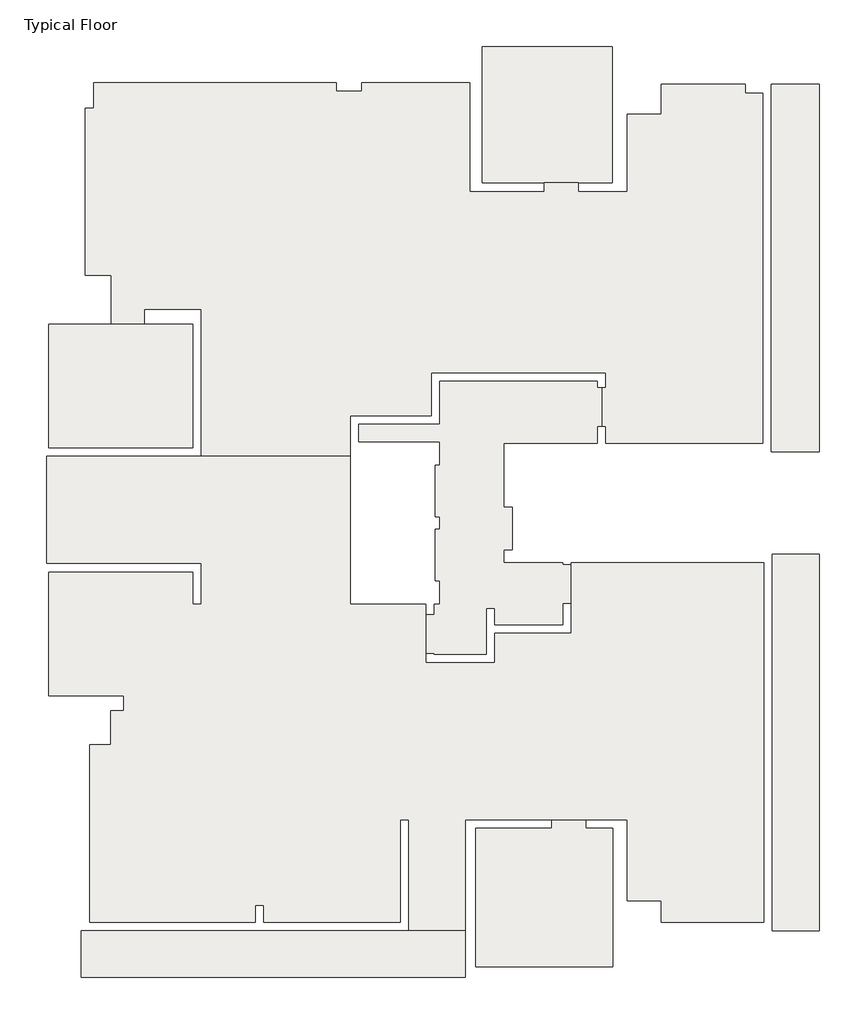
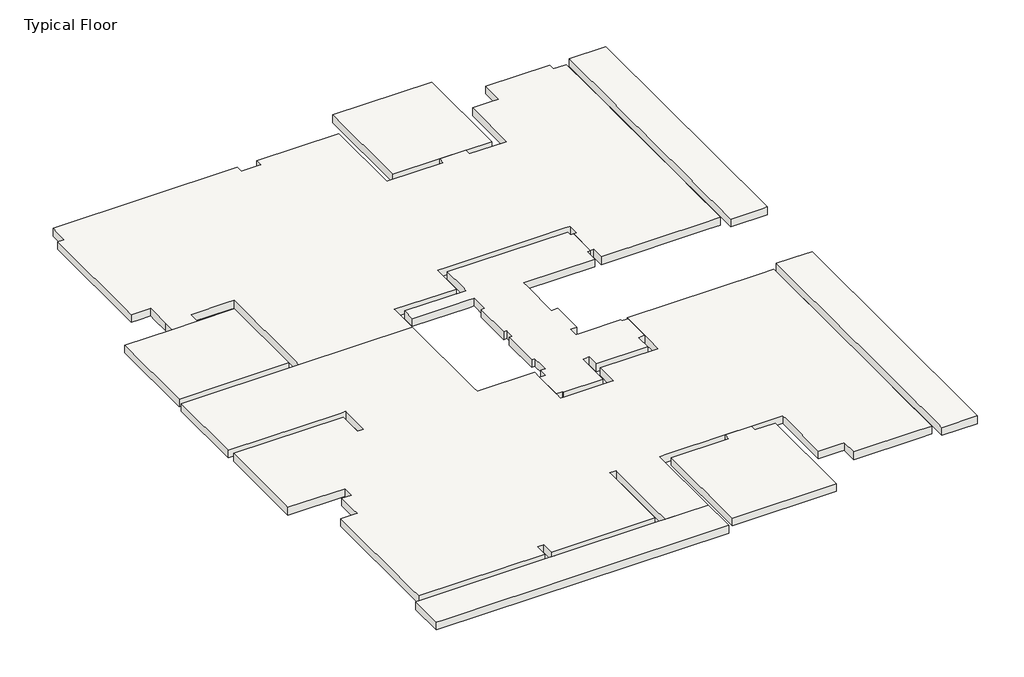
# One storey: 9 slabs.
"""IFC4 building model written with IfcOpenShell, lengths in millimetres."""

from ifc_helpers import new_model, si_unit, frame, origin, place, context, project, spatial, polyline, outline, extrude, faceted_brep, element, save

model = new_model("IFC4")

# Units and contexts
model_context = context("Model", 3, world=origin())
ifc_project = project(units=[si_unit("LENGTHUNIT", "METRE", prefix="MILLI")], contexts=[model_context])

# Site, building, storey
site = spatial("IfcSite", under=ifc_project)
building = spatial("IfcBuilding", under=site)
storey = spatial("IfcBuildingStorey", under=building, Name="Typical Floor", Elevation=3150.0)

# Slabs
placement = place(None, origin())
element("IfcSlab", 1, ObjectType="25", at=placement, inside=storey, context=model_context, shape_type="Brep", body=[
    faceted_brep([(1799.9138343, 9657.4646681, 2900.0), (1799.9138343, 6457.4646681, 2900.0), (1000.2209526, 6457.4646681, 2900.0), (199.8822614, 6457.4646681, 2900.0), (-1246.8886915, 6457.4646681, 2900.0), (-1246.8886915, 9657.4646681, 2900.0), (1799.9138343, 9657.4646681, 3150.0), (-1246.8886915, 9657.4646681, 3150.0), (-1246.8886915, 6457.4646681, 3150.0), (199.8822614, 6457.4646681, 3150.0), (1000.2209526, 6457.4646681, 3150.0), (1799.9138343, 6457.4646681, 3150.0)], [[[0, 1, 2, 3, 4, 5]], [[6, 7, 8, 9, 10, 11]], [[1, 0, 6, 11]], [[4, 3, 2, 1, 11, 10, 9, 8]], [[5, 4, 8, 7]], [[0, 5, 7, 6]]]),
])
element("IfcSlab", 2, ObjectType="25", at=placement, inside=storey, context=model_context, shape_type="Brep", body=[
    faceted_brep([(-8041.6160164, 3148.6252115, 2900.0), (-8041.6160164, 247.4292682, 2900.0), (-11417.5737279, 247.4292682, 2900.0), (-11417.5737279, 3148.6252115, 2900.0), (-9955.8228668, 3148.6252115, 2900.0), (-9181.8657294, 3148.6252115, 2900.0), (-8041.6160164, 3148.6252115, 3150.0), (-9181.8657294, 3148.6252115, 3150.0), (-9955.8228668, 3148.6252115, 3150.0), (-11417.5737279, 3148.6252115, 3150.0), (-11417.5737279, 247.4292682, 3150.0), (-8041.6160164, 247.4292682, 3150.0)], [[[0, 1, 2, 3, 4, 5]], [[6, 7, 8, 9, 10, 11]], [[1, 0, 6, 11]], [[2, 1, 11, 10]], [[3, 2, 10, 9]], [[0, 5, 4, 3, 9, 8, 7, 6]]]),
])
element("IfcSlab", 3, ObjectType="25", at=placement, inside=storey, context=model_context, shape_type="Brep", body=[
    faceted_brep([(-11467.5737279, -2465.8036059, 2900.0), (-11467.5737279, 47.4292682, 2900.0), (-7841.6160164, 47.4292682, 2900.0), (-4348.0741106, 47.4292682, 2900.0), (-4348.0741106, -3216.4704639, 2900.0), (-4348.0741106, -3416.4704639, 2900.0), (-2578.9868545, -3416.4704639, 2900.0), (-2578.9868545, -3670.5462389, 2900.0), (-2578.9868545, -4570.3979419, 2900.0), (-2578.9868545, -4796.9488413, 2900.0), (-2378.9868545, -4796.9488413, 2900.0), (-951.9279184, -4796.9488413, 2900.0), (-951.9279184, -4596.9488413, 2900.0), (-951.9279184, -4098.2404601, 2900.0), (833.928377, -4098.2404601, 2900.0), (833.928377, -3898.2404601, 2900.0), (833.928377, -3399.5320789, 2900.0), (833.928377, -2499.6803759, 2900.0), (833.928377, -2446.7479228, 2900.0), (4951.7310336, -2446.7479228, 2900.0), (5351.7310336, -2446.7479228, 2900.0), (5351.7310336, -10874.7377812, 2900.0), (4951.7310336, -10874.7377812, 2900.0), (2953.3437999, -10874.7377812, 2900.0), (2953.3437999, -10374.7377812, 2900.0), (2753.3437999, -10374.7377812, 2900.0), (2155.1912932, -10374.7377812, 2900.0), (2155.1912932, -8672.5783859, 2900.0), (2155.1912932, -8472.5783859, 2900.0), (1180.1912932, -8472.5783859, 2900.0), (379.852602, -8472.5783859, 2900.0), (-1396.4017034, -8472.5783859, 2900.0), (-1646.4017034, -8472.5783859, 2900.0), (-1646.4017034, -11075.5031849, 2900.0), (-2972.9736513, -11075.5031849, 2900.0), (-2972.9736513, -10475.5031849, 2900.0), (-2972.9736513, -9073.8910533, 2900.0), (-2972.9736513, -8473.8910533, 2900.0), (-3172.9736513, -8473.8910533, 2900.0), (-3172.9736513, -9073.8910533, 2900.0), (-3172.9736513, -10475.5031849, 2900.0), (-3172.9736513, -10874.7377812, 2900.0), (-6376.4457141, -10874.7377812, 2900.0), (-6376.4457141, -10475.5031849, 2900.0), (-6576.4457141, -10475.5031849, 2900.0), (-6576.4457141, -10874.7377812, 2900.0), (-10457.6225223, -10874.7377812, 2900.0), (-10457.6225223, -10475.5031849, 2900.0), (-10457.6225223, -6721.9995493, 2900.0), (-9957.6225223, -6721.9995493, 2900.0), (-9957.6225223, -6521.9995493, 2900.0), (-9957.6225223, -5916.9995493, 2900.0), (-9656.1405093, -5916.9995493, 2900.0), (-9656.1405093, -5566.9995493, 2900.0), (-11417.5737279, -5566.9995493, 2900.0), (-11417.5737279, -2665.8036059, 2900.0), (-8042.7593383, -2665.8036059, 2900.0), (-8042.7593383, -3416.4704639, 2900.0), (-7842.7593383, -3416.4704639, 2900.0), (-7842.7593383, -2465.8036059, 2900.0), (-8042.7593383, -2465.8036059, 2900.0), (-11467.5737279, 47.4292682, 3150.0), (-11467.5737279, -2465.8036059, 3150.0), (-8042.7593383, -2465.8036059, 3150.0), (-7842.7593383, -2465.8036059, 3150.0), (-7842.7593383, -3416.4704639, 3150.0), (-8042.7593383, -3416.4704639, 3150.0), (-8042.7593383, -2665.8036059, 3150.0), (-11417.5737279, -2665.8036059, 3150.0), (-11417.5737279, -5566.9995493, 3150.0), (-9656.1405093, -5566.9995493, 3150.0), (-9656.1405093, -5916.9995493, 3150.0), (-9957.6225223, -5916.9995493, 3150.0), (-9957.6225223, -6521.9995493, 3150.0), (-9957.6225223, -6721.9995493, 3150.0), (-10457.6225223, -6721.9995493, 3150.0), (-10457.6225223, -10475.5031849, 3150.0), (-10457.6225223, -10874.7377812, 3150.0), (-6576.4457141, -10874.7377812, 3150.0), (-6576.4457141, -10475.5031849, 3150.0), (-6376.4457141, -10475.5031849, 3150.0), (-6376.4457141, -10874.7377812, 3150.0), (-3172.9736513, -10874.7377812, 3150.0), (-3172.9736513, -10475.5031849, 3150.0), (-3172.9736513, -9073.8910533, 3150.0), (-3172.9736513, -8473.8910533, 3150.0), (-2972.9736513, -8473.8910533, 3150.0), (-2972.9736513, -9073.8910533, 3150.0), (-2972.9736513, -10475.5031849, 3150.0), (-2972.9736513, -11075.5031849, 3150.0), (-1646.4017034, -11075.5031849, 3150.0), (-1646.4017034, -8472.5783859, 3150.0), (-1396.4017034, -8472.5783859, 3150.0), (379.852602, -8472.5783859, 3150.0), (1180.1912932, -8472.5783859, 3150.0), (2155.1912932, -8472.5783859, 3150.0), (2155.1912932, -8672.5783859, 3150.0), (2155.1912932, -10374.7377812, 3150.0), (2753.3437999, -10374.7377812, 3150.0), (2953.3437999, -10374.7377812, 3150.0), (2953.3437999, -10874.7377812, 3150.0), (4951.7310336, -10874.7377812, 3150.0), (5351.7310336, -10874.7377812, 3150.0), (5351.7310336, -9023.8910533, 3150.0), (5351.7310336, -8523.8910533, 3150.0), (5351.7310336, -4555.4465944, 3150.0), (5351.7310336, -4055.4465944, 3150.0), (5351.7310336, -2446.7479228, 3150.0), (4951.7310336, -2446.7479228, 3150.0), (833.928377, -2446.7479228, 3150.0), (833.928377, -2499.6803759, 3150.0), (833.928377, -3399.5320789, 3150.0), (833.928377, -3898.2404601, 3150.0), (833.928377, -4098.2404601, 3150.0), (-951.9279184, -4098.2404601, 3150.0), (-951.9279184, -4596.9488413, 3150.0), (-951.9279184, -4796.9488413, 3150.0), (-2378.9868545, -4796.9488413, 3150.0), (-2578.9868545, -4796.9488413, 3150.0), (-2578.9868545, -4570.3979419, 3150.0), (-2578.9868545, -3670.5462389, 3150.0), (-2578.9868545, -3416.4704639, 3150.0), (-4348.0741106, -3416.4704639, 3150.0), (-4348.0741106, -3216.4704639, 3150.0), (-4348.0741106, 47.4292682, 3150.0), (-7841.6160164, 47.4292682, 3150.0)], [[[0, 1, 2, 3, 4, 5, 6, 7, 8, 9, 10, 11, 12, 13, 14, 15, 16, 17, 18, 19, 20, 21, 22, 23, 24, 25, 26, 27, 28, 29, 30, 31, 32, 33, 34, 35, 36, 37, 38, 39, 40, 41, 42, 43, 44, 45, 46, 47, 48, 49, 50, 51, 52, 53, 54, 55, 56, 57, 58, 59, 60]], [[61, 62, 63, 64, 65, 66, 67, 68, 69, 70, 71, 72, 73, 74, 75, 76, 77, 78, 79, 80, 81, 82, 83, 84, 85, 86, 87, 88, 89, 90, 91, 92, 93, 94, 95, 96, 97, 98, 99, 100, 101, 102, 103, 104, 105, 106, 107, 108, 109, 110, 111, 112, 113, 114, 115, 116, 117, 118, 119, 120, 121, 122, 123, 124, 125]], [[1, 0, 62, 61]], [[2, 1, 61, 125]], [[3, 2, 125, 124]], [[3, 124, 123, 122, 5, 4]], [[6, 5, 122, 121]], [[6, 121, 120, 119, 118, 9, 8, 7]], [[9, 118, 117, 116, 11, 10]], [[11, 116, 115, 114, 13, 12]], [[14, 13, 114, 113]], [[14, 113, 112, 111, 110, 109, 18, 17, 16, 15]], [[18, 109, 108, 107, 20, 19]], [[21, 20, 107, 106, 105, 104, 103, 102]], [[21, 102, 101, 100, 23, 22]], [[24, 23, 100, 99]], [[24, 99, 98, 97, 26, 25]], [[26, 97, 96, 95, 28, 27]], [[28, 95, 94, 93, 92, 91, 32, 31, 30, 29]], [[33, 32, 91, 90]], [[34, 33, 90, 89]], [[34, 89, 88, 87, 86, 37, 36, 35]], [[38, 37, 86, 85]], [[38, 85, 84, 83, 82, 41, 40, 39]], [[42, 41, 82, 81]], [[43, 42, 81, 80]], [[44, 43, 80, 79]], [[45, 44, 79, 78]], [[46, 45, 78, 77]], [[46, 77, 76, 75, 48, 47]], [[49, 48, 75, 74]], [[49, 74, 73, 72, 51, 50]], [[52, 51, 72, 71]], [[53, 52, 71, 70]], [[54, 53, 70, 69]], [[55, 54, 69, 68]], [[56, 55, 68, 67]], [[57, 56, 67, 66]], [[58, 57, 66, 65]], [[59, 58, 65, 64]], [[59, 64, 63, 62, 0, 60]]]),
])
element("IfcSlab", 4, ObjectType="25", at=placement, inside=storey, context=model_context, shape_type="Brep", body=[
    faceted_brep([(-2578.9868545, -4570.3979419, 2900.0), (-2578.9868545, -3670.5462389, 2900.0), (-2378.9868545, -3670.5462389, 2900.0), (-2378.9868545, -3416.4704639, 2900.0), (-2247.7143708, -3416.4704639, 2900.0), (-2247.7143708, -3216.4704639, 2900.0), (-2247.7143708, -2865.9729515, 2900.0), (-2347.7143708, -2865.9729515, 2900.0), (-2347.7143708, -1665.4649148, 2900.0), (-2247.7143708, -1665.4649148, 2900.0), (-2247.7143708, -1366.9258792, 2900.0), (-2347.7143708, -1366.9258792, 2900.0), (-2347.7143708, -166.4178424, 2900.0), (-2247.7143708, -166.4178424, 2900.0), (-2247.7143708, 384.07967, 2900.0), (-2447.7143708, 384.07967, 2900.0), (-4148.0741106, 384.07967, 2900.0), (-4148.0741106, 794.07967, 2900.0), (-2249.8316689, 794.07967, 2900.0), (-2249.8316689, 994.07967, 2900.0), (-2249.8316689, 1803.8127355, 2900.0), (1452.348775, 1803.8127355, 2900.0), (1452.348775, 1652.3412467, 2900.0), (1552.348775, 1652.3412467, 2900.0), (1552.348775, 750.3722456, 2900.0), (1452.348775, 750.3722456, 2900.0), (1452.348775, 352.3201981, 2900.0), (-748.6672985, 352.3201981, 2900.0), (-748.6672985, 152.3201981, 2900.0), (-748.6672985, -1148.8441723, 2900.0), (-548.6672985, -1148.8441723, 2900.0), (-548.6672985, -2148.2088872, 2900.0), (-748.6672985, -2148.2088872, 2900.0), (-748.6672985, -2446.7479228, 2900.0), (-548.6672985, -2446.7479228, 2900.0), (633.928377, -2446.7479228, 2900.0), (633.928377, -2499.6803759, 2900.0), (833.928377, -2499.6803759, 2900.0), (833.928377, -3399.5320789, 2900.0), (633.928377, -3399.5320789, 2900.0), (633.928377, -3898.2404601, 2900.0), (-951.9279184, -3898.2404601, 2900.0), (-951.9279184, -3515.9834758, 2900.0), (-1151.9279184, -3515.9834758, 2900.0), (-1151.9279184, -4596.9488413, 2900.0), (-2378.9868545, -4596.9488413, 2900.0), (-2378.9868545, -4570.3979419, 2900.0), (-2578.9868545, -3670.5462389, 3150.0), (-2578.9868545, -4570.3979419, 3150.0), (-2378.9868545, -4570.3979419, 3150.0), (-2378.9868545, -4596.9488413, 3150.0), (-1151.9279184, -4596.9488413, 3150.0), (-1151.9279184, -3515.9834758, 3150.0), (-951.9279184, -3515.9834758, 3150.0), (-951.9279184, -3898.2404601, 3150.0), (633.928377, -3898.2404601, 3150.0), (633.928377, -3399.5320789, 3150.0), (833.928377, -3399.5320789, 3150.0), (833.928377, -2499.6803759, 3150.0), (633.928377, -2499.6803759, 3150.0), (633.928377, -2446.7479228, 3150.0), (-548.6672985, -2446.7479228, 3150.0), (-748.6672985, -2446.7479228, 3150.0), (-748.6672985, -2148.2088872, 3150.0), (-548.6672985, -2148.2088872, 3150.0), (-548.6672985, -1148.8441723, 3150.0), (-748.6672985, -1148.8441723, 3150.0), (-748.6672985, 152.3201981, 3150.0), (-748.6672985, 352.3201981, 3150.0), (1452.348775, 352.3201981, 3150.0), (1452.348775, 750.3722456, 3150.0), (1552.348775, 750.3722456, 3150.0), (1552.348775, 1652.3412467, 3150.0), (1452.348775, 1652.3412467, 3150.0), (1452.348775, 1803.8127355, 3150.0), (-2249.8316689, 1803.8127355, 3150.0), (-2249.8316689, 994.07967, 3150.0), (-2249.8316689, 794.07967, 3150.0), (-4148.0741106, 794.07967, 3150.0), (-4148.0741106, 384.07967, 3150.0), (-2447.7143708, 384.07967, 3150.0), (-2247.7143708, 384.07967, 3150.0), (-2247.7143708, -166.4178424, 3150.0), (-2347.7143708, -166.4178424, 3150.0), (-2347.7143708, -1366.9258792, 3150.0), (-2247.7143708, -1366.9258792, 3150.0), (-2247.7143708, -1665.4649148, 3150.0), (-2347.7143708, -1665.4649148, 3150.0), (-2347.7143708, -2865.9729515, 3150.0), (-2247.7143708, -2865.9729515, 3150.0), (-2247.7143708, -3216.4704639, 3150.0), (-2247.7143708, -3416.4704639, 3150.0), (-2378.9868545, -3416.4704639, 3150.0), (-2378.9868545, -3670.5462389, 3150.0)], [[[0, 1, 2, 3, 4, 5, 6, 7, 8, 9, 10, 11, 12, 13, 14, 15, 16, 17, 18, 19, 20, 21, 22, 23, 24, 25, 26, 27, 28, 29, 30, 31, 32, 33, 34, 35, 36, 37, 38, 39, 40, 41, 42, 43, 44, 45, 46]], [[47, 48, 49, 50, 51, 52, 53, 54, 55, 56, 57, 58, 59, 60, 61, 62, 63, 64, 65, 66, 67, 68, 69, 70, 71, 72, 73, 74, 75, 76, 77, 78, 79, 80, 81, 82, 83, 84, 85, 86, 87, 88, 89, 90, 91, 92, 93]], [[1, 0, 48, 47]], [[2, 1, 47, 93]], [[3, 2, 93, 92]], [[4, 3, 92, 91]], [[4, 91, 90, 89, 6, 5]], [[7, 6, 89, 88]], [[8, 7, 88, 87]], [[9, 8, 87, 86]], [[10, 9, 86, 85]], [[11, 10, 85, 84]], [[12, 11, 84, 83]], [[13, 12, 83, 82]], [[14, 13, 82, 81]], [[14, 81, 80, 79, 16, 15]], [[17, 16, 79, 78]], [[18, 17, 78, 77]], [[18, 77, 76, 75, 20, 19]], [[21, 20, 75, 74]], [[22, 21, 74, 73]], [[23, 22, 73, 72]], [[24, 23, 72, 71]], [[25, 24, 71, 70]], [[26, 25, 70, 69]], [[27, 26, 69, 68]], [[27, 68, 67, 66, 29, 28]], [[30, 29, 66, 65]], [[31, 30, 65, 64]], [[32, 31, 64, 63]], [[33, 32, 63, 62]], [[33, 62, 61, 60, 35, 34]], [[36, 35, 60, 59]], [[37, 36, 59, 58]], [[38, 37, 58, 57]], [[39, 38, 57, 56]], [[40, 39, 56, 55]], [[41, 40, 55, 54]], [[42, 41, 54, 53]], [[43, 42, 53, 52]], [[44, 43, 52, 51]], [[45, 44, 51, 50]], [[46, 45, 50, 49]], [[0, 46, 49, 48]]]),
])
element("IfcSlab", 5, ObjectType="25", at=placement, inside=storey, context=model_context, shape_type="Brep", body=[
    faceted_brep([(-1546.8886915, 6257.4646681, 2900.0), (199.8822614, 6257.4646681, 2900.0), (199.8822614, 6457.4646681, 2900.0), (1000.2209526, 6457.4646681, 2900.0), (1000.2209526, 6257.4646681, 2900.0), (2149.9138343, 6257.4646681, 2900.0), (2149.9138343, 6457.4646681, 2900.0), (2149.9138343, 8067.4646681, 2900.0), (2753.3437999, 8067.4646681, 2900.0), (2953.3437999, 8067.4646681, 2900.0), (2953.3437999, 8567.4646681, 2900.0), (2953.3437999, 8767.4646681, 2900.0), (4922.8790959, 8767.4646681, 2900.0), (4922.8790959, 8567.4646681, 2900.0), (5322.8790959, 8567.4646681, 2900.0), (5322.8790959, 352.3201981, 2900.0), (4922.8790959, 352.3201981, 2900.0), (1652.348775, 352.3201981, 2900.0), (1652.348775, 750.3722456, 2900.0), (1552.348775, 750.3722456, 2900.0), (1552.348775, 1652.3412467, 2900.0), (1652.348775, 1652.3412467, 2900.0), (1652.348775, 2003.8127355, 2900.0), (1452.348775, 2003.8127355, 2900.0), (-2249.8316689, 2003.8127355, 2900.0), (-2449.8316689, 2003.8127355, 2900.0), (-2449.8316689, 994.07967, 2900.0), (-4348.0741106, 994.07967, 2900.0), (-4348.0741106, 794.07967, 2900.0), (-4348.0741106, 47.4292682, 2900.0), (-7841.6160164, 47.4292682, 2900.0), (-7841.6160164, 247.4292682, 2900.0), (-7841.6160164, 3498.6252115, 2900.0), (-8041.6160164, 3498.6252115, 2900.0), (-9181.8657294, 3498.6252115, 2900.0), (-9181.8657294, 3148.6252115, 2900.0), (-9955.8228668, 3148.6252115, 2900.0), (-9955.8228668, 3498.6252115, 2900.0), (-9955.8228668, 4097.8205808, 2900.0), (-9955.8228668, 4297.8205808, 2900.0), (-10355.9922124, 4297.8205808, 2900.0), (-10555.8228668, 4297.8205808, 2900.0), (-10555.9922124, 4297.8205808, 2900.0), (-10555.9922124, 8213.0435047, 2900.0), (-10355.9922124, 8213.0435047, 2900.0), (-10355.9922124, 8813.0435047, 2900.0), (-4673.6985753, 8813.0435047, 2900.0), (-4673.6985753, 8613.0435047, 2900.0), (-4073.6985753, 8613.0435047, 2900.0), (-4073.6985753, 8813.0435047, 2900.0), (-1546.8886915, 8813.0435047, 2900.0), (-1546.8886915, 6457.4646681, 2900.0), (199.8822614, 6257.4646681, 3150.0), (-1546.8886915, 6257.4646681, 3150.0), (-1546.8886915, 6457.4646681, 3150.0), (-1546.8886915, 8613.0435047, 3150.0), (-1546.8886915, 8813.0435047, 3150.0), (-4073.6985753, 8813.0435047, 3150.0), (-4073.6985753, 8613.0435047, 3150.0), (-4673.6985753, 8613.0435047, 3150.0), (-4673.6985753, 8813.0435047, 3150.0), (-10355.9922124, 8813.0435047, 3150.0), (-10355.9922124, 8613.0435047, 3150.0), (-10355.9922124, 8213.0435047, 3150.0), (-10555.9922124, 8213.0435047, 3150.0), (-10555.9922124, 4297.8205808, 3150.0), (-10555.8228668, 4297.8205808, 3150.0), (-9955.8228668, 4297.8205808, 3150.0), (-9955.8228668, 4097.8205808, 3150.0), (-9955.8228668, 3498.6252115, 3150.0), (-9955.8228668, 3148.6252115, 3150.0), (-9181.8657294, 3148.6252115, 3150.0), (-9181.8657294, 3498.6252115, 3150.0), (-8041.6160164, 3498.6252115, 3150.0), (-7841.6160164, 3498.6252115, 3150.0), (-7841.6160164, 247.4292682, 3150.0), (-7841.6160164, 47.4292682, 3150.0), (-4348.0741106, 47.4292682, 3150.0), (-4348.0741106, 794.07967, 3150.0), (-4348.0741106, 994.07967, 3150.0), (-2449.8316689, 994.07967, 3150.0), (-2449.8316689, 2003.8127355, 3150.0), (-2249.8316689, 2003.8127355, 3150.0), (1452.348775, 2003.8127355, 3150.0), (1652.348775, 2003.8127355, 3150.0), (1652.348775, 1652.3412467, 3150.0), (1552.348775, 1652.3412467, 3150.0), (1552.348775, 750.3722456, 3150.0), (1652.348775, 750.3722456, 3150.0), (1652.348775, 352.3201981, 3150.0), (4922.8790959, 352.3201981, 3150.0), (5322.8790959, 352.3201981, 3150.0), (5322.8790959, 1946.2717251, 3150.0), (5322.8790959, 2446.2717251, 3150.0), (5322.8790959, 6003.9942904, 3150.0), (5322.8790959, 6503.9942904, 3150.0), (5322.8790959, 8567.4646681, 3150.0), (4922.8790959, 8567.4646681, 3150.0), (4922.8790959, 8767.4646681, 3150.0), (2953.3437999, 8767.4646681, 3150.0), (2953.3437999, 8067.4646681, 3150.0), (2753.3437999, 8067.4646681, 3150.0), (2149.9138343, 8067.4646681, 3150.0), (2149.9138343, 6457.4646681, 3150.0), (2149.9138343, 6257.4646681, 3150.0), (1000.2209526, 6257.4646681, 3150.0), (1000.2209526, 6457.4646681, 3150.0), (199.8822614, 6457.4646681, 3150.0)], [[[0, 1, 2, 3, 4, 5, 6, 7, 8, 9, 10, 11, 12, 13, 14, 15, 16, 17, 18, 19, 20, 21, 22, 23, 24, 25, 26, 27, 28, 29, 30, 31, 32, 33, 34, 35, 36, 37, 38, 39, 40, 41, 42, 43, 44, 45, 46, 47, 48, 49, 50, 51]], [[52, 53, 54, 55, 56, 57, 58, 59, 60, 61, 62, 63, 64, 65, 66, 67, 68, 69, 70, 71, 72, 73, 74, 75, 76, 77, 78, 79, 80, 81, 82, 83, 84, 85, 86, 87, 88, 89, 90, 91, 92, 93, 94, 95, 96, 97, 98, 99, 100, 101, 102, 103, 104, 105, 106, 107]], [[42, 65, 64, 43]], [[56, 50, 49, 57]], [[45, 61, 60, 46]], [[50, 56, 55, 54, 53, 0, 51]], [[1, 0, 53, 52]], [[2, 1, 52, 107]], [[3, 2, 107, 106]], [[4, 3, 106, 105]], [[5, 4, 105, 104]], [[5, 104, 103, 102, 7, 6]], [[8, 7, 102, 101]], [[9, 8, 101, 100]], [[11, 10, 9, 100, 99]], [[11, 99, 98, 12]], [[91, 15, 14, 96, 95, 94, 93, 92]], [[15, 91, 90, 89, 17, 16]], [[18, 17, 89, 88]], [[19, 18, 88, 87]], [[20, 19, 87, 86]], [[21, 20, 86, 85]], [[22, 21, 85, 84]], [[22, 84, 83, 82, 81, 25, 24, 23]], [[26, 25, 81, 80]], [[27, 26, 80, 79]], [[27, 79, 78, 77, 29, 28]], [[30, 29, 77, 76]], [[30, 76, 75, 74, 32, 31]], [[37, 36, 70, 69]], [[37, 69, 68, 67, 39, 38]], [[39, 67, 66, 65, 42, 41, 40]], [[44, 63, 62, 61, 45]], [[63, 44, 43, 64]], [[48, 58, 57, 49]], [[58, 48, 47, 59]], [[59, 47, 46, 60]], [[13, 97, 96, 14]], [[97, 13, 12, 98]], [[32, 74, 73, 72, 34, 33]], [[35, 34, 72, 71]], [[36, 35, 71, 70]]]),
])
element("IfcSlab", 6, ObjectType="25", at=placement, inside=storey, context=model_context, shape_type="SweptSolid", body=[
    extrude(outline(polyline([(379.852602, -8672.5783859), (379.852602, -8472.5783859), (1180.1912932, -8472.5783859), (1180.1912932, -8672.5783859), (1805.1912932, -8672.5783859), (1805.1912932, -11923.6155079), (-1396.4017034, -11923.6155079), (-1396.4017034, -8672.5783859), (379.852602, -8672.5783859)])), frame((0.0, 0.0, 2900.0), z_axis=(0.0, 0.0, 1.0), x_axis=(1.0, 0.0, 0.0)), (0.0, 0.0, 1.0), 250.0),
])
element("IfcSlab", 7, ObjectType="25", at=placement, inside=storey, context=model_context, shape_type="Brep", body=[
    faceted_brep([(-1646.4017034, -12173.6155079, 2900.0), (-10657.6225223, -12173.6155079, 2900.0), (-10657.6225223, -11075.5031849, 2900.0), (-10457.6225223, -11075.5031849, 2900.0), (-10457.6225223, -11074.7377812, 2900.0), (-10457.6225223, -11073.8349319, 2900.0), (-6576.4457141, -11073.8349319, 2900.0), (-6576.4457141, -11074.7377812, 2900.0), (-6576.4457141, -11075.5031849, 2900.0), (-6376.4457141, -11075.5031849, 2900.0), (-6376.4457141, -11074.7377812, 2900.0), (-6376.4457141, -11073.8349319, 2900.0), (-3172.9736513, -11073.8349319, 2900.0), (-3172.9736513, -11074.7377812, 2900.0), (-3172.9736513, -11075.5031849, 2900.0), (-2972.9736513, -11075.5031849, 2900.0), (-1646.4017034, -11075.5031849, 2900.0), (-10657.6225223, -12173.6155079, 3150.0), (-10457.6225223, -12173.6155079, 3150.0), (-1646.4017034, -12173.6155079, 3150.0), (-1646.4017034, -11973.6155079, 3150.0), (-1646.4017034, -11075.5031849, 3150.0), (-2972.9736513, -11075.5031849, 3150.0), (-3172.9736513, -11075.5031849, 3150.0), (-3172.9736513, -11073.8349319, 3150.0), (-6376.4457141, -11073.8349319, 3150.0), (-6376.4457141, -11075.5031849, 3150.0), (-6576.4457141, -11075.5031849, 3150.0), (-6576.4457141, -11073.8349319, 3150.0), (-10457.6225223, -11073.8349319, 3150.0), (-10457.6225223, -11075.5031849, 3150.0), (-10657.6225223, -11075.5031849, 3150.0)], [[[0, 1, 2, 3, 4, 5, 6, 7, 8, 9, 10, 11, 12, 13, 14, 15, 16]], [[17, 18, 19, 20, 21, 22, 23, 24, 25, 26, 27, 28, 29, 30, 31]], [[19, 0, 16, 21, 20]], [[1, 0, 19, 18, 17]], [[1, 17, 31, 2]], [[5, 29, 28, 6]], [[11, 25, 24, 12]], [[3, 30, 29, 5, 4]], [[30, 3, 2, 31]], [[9, 26, 25, 11, 10]], [[26, 9, 8, 27]], [[27, 8, 7, 6, 28]], [[14, 23, 22, 21, 16, 15]], [[23, 14, 13, 12, 24]]]),
])
element("IfcSlab", 8, ObjectType="25", at=placement, inside=storey, context=model_context, shape_type="Brep", body=[
    faceted_brep([(6650.1463257, 152.3201981, 2900.0), (5522.8790959, 152.3201981, 2900.0), (5522.8790959, 8767.4646681, 2900.0), (6650.1463257, 8767.4646681, 2900.0), (6650.1463257, 152.3201981, 3150.0), (6650.1463257, 8567.4646681, 3150.0), (6650.1463257, 8767.4646681, 3150.0), (5522.8790959, 8767.4646681, 3150.0), (5522.8790959, 8567.4646681, 3150.0), (5522.8790959, 6503.9942904, 3150.0), (5522.8790959, 6003.9942904, 3150.0), (5522.8790959, 2446.2717251, 3150.0), (5522.8790959, 1946.2717251, 3150.0), (5522.8790959, 352.3201981, 3150.0), (5522.8790959, 152.3201981, 3150.0), (6450.1463257, 152.3201981, 3150.0)], [[[0, 1, 2, 3]], [[4, 5, 6, 7, 8, 9, 10, 11, 12, 13, 14, 15]], [[1, 0, 4, 15, 14]], [[2, 1, 14, 13, 12, 11, 10, 9, 8, 7]], [[3, 2, 7, 6]], [[0, 3, 6, 5, 4]]]),
])
element("IfcSlab", 9, ObjectType="25", at=placement, inside=storey, context=model_context, shape_type="Brep", body=[
    faceted_brep([(6650.1463257, -11074.7377812, 2900.0), (5551.7310336, -11074.7377812, 2900.0), (5551.7310336, -2246.7479228, 2900.0), (6650.1463257, -2246.7479228, 2900.0), (6650.1463257, -11074.7377812, 3150.0), (6650.1463257, -10874.7377812, 3150.0), (6650.1463257, -2246.7479228, 3150.0), (6450.1463257, -2246.7479228, 3150.0), (5551.7310336, -2246.7479228, 3150.0), (5551.7310336, -2446.7479228, 3150.0), (5551.7310336, -4055.4465944, 3150.0), (5551.7310336, -4555.4465944, 3150.0), (5551.7310336, -8523.8910533, 3150.0), (5551.7310336, -9023.8910533, 3150.0), (5551.7310336, -10874.7377812, 3150.0), (5551.7310336, -11074.7377812, 3150.0)], [[[0, 1, 2, 3]], [[4, 5, 6, 7, 8, 9, 10, 11, 12, 13, 14, 15]], [[1, 0, 4, 15]], [[2, 1, 15, 14, 13, 12, 11, 10, 9, 8]], [[3, 2, 8, 7, 6]], [[0, 3, 6, 5, 4]]]),
])

save(model, "model.ifc")

# Revit data of these elements
# Type "25"
#   Function = 0
#   Layers, outside or top first: 25 cm "Concrete" (function 1)
# Element 1 (IfcSlab, "25")
#   Mark = "S1"
#   SOFiSTiK_AMG_Comments = ""
#   Height Offset From Level = 0 cm
#   built-in parameter 1001954 = 1
#   SOFiSTiK_AMG_Scheduled = yes
#   SOFiSTiK_AMG_Adjusted = yes
#   Phase Created = New Construction
#   Materials on its faces: "Concrete"
# Element 2 (IfcSlab, "25")
#   Mark = "S2"
#   SOFiSTiK_AMG_Comments = ""
#   Height Offset From Level = 0 cm
#   built-in parameter 1001954 = 1
#   SOFiSTiK_AMG_Scheduled = yes
#   SOFiSTiK_AMG_Adjusted = yes
#   Phase Created = New Construction
#   Materials on its faces: "Concrete"
# Element 3 (IfcSlab, "25")
#   Mark = "S3"
#   SOFiSTiK_AMG_Comments = ""
#   built-in parameter 1001955 = -1.5708 (stored number, unit not read)
#   Height Offset From Level = 0 cm
#   built-in parameter 1001954 = 1
#   SOFiSTiK_AMG_Scheduled = yes
#   SOFiSTiK_AMG_Adjusted = no
#   Phase Created = New Construction
#   Materials on its faces: "Concrete"
# Element 4 (IfcSlab, "25")
#   Mark = "S4"
#   SOFiSTiK_AMG_Comments = ""
#   built-in parameter 1001955 = -1.5708 (stored number, unit not read)
#   Height Offset From Level = 0 cm
#   built-in parameter 1001954 = 1
#   SOFiSTiK_AMG_Scheduled = yes
#   SOFiSTiK_AMG_Adjusted = yes
#   Phase Created = New Construction
#   Materials on its faces: "Concrete"
# Element 5 (IfcSlab, "25")
#   Mark = "S5"
#   SOFiSTiK_AMG_Comments = ""
#   built-in parameter 1001955 = -1.5708 (stored number, unit not read)
#   Height Offset From Level = 0 cm
#   built-in parameter 1001954 = 1
#   SOFiSTiK_AMG_Scheduled = yes
#   SOFiSTiK_AMG_Adjusted = yes
#   Phase Created = New Construction
#   Materials on its faces: "Concrete"
# Element 6 (IfcSlab, "25")
#   Mark = "S6"
#   SOFiSTiK_AMG_Comments = ""
#   Height Offset From Level = 0 cm
#   built-in parameter 1001954 = 1
#   SOFiSTiK_AMG_Scheduled = yes
#   SOFiSTiK_AMG_Adjusted = yes
#   Phase Created = New Construction
#   Materials on its faces: "Concrete"
# Element 7 (IfcSlab, "25")
#   Mark = "S7"
#   SOFiSTiK_AMG_Comments = ""
#   Height Offset From Level = 0 cm
#   built-in parameter 1001954 = 1
#   SOFiSTiK_AMG_Scheduled = yes
#   SOFiSTiK_AMG_Adjusted = yes
#   Phase Created = New Construction
#   Materials on its faces: "Concrete"
# Element 8 (IfcSlab, "25")
#   Mark = "S8"
#   SOFiSTiK_AMG_Comments = ""
#   Height Offset From Level = 0 cm
#   built-in parameter 1001954 = 1
#   SOFiSTiK_AMG_Scheduled = yes
#   SOFiSTiK_AMG_Adjusted = yes
#   Phase Created = New Construction
#   Materials on its faces: "Concrete"
# Element 9 (IfcSlab, "25")
#   Mark = "S9"
#   SOFiSTiK_AMG_Comments = ""
#   Height Offset From Level = 0 cm
#   built-in parameter 1001954 = 1
#   SOFiSTiK_AMG_Scheduled = yes
#   SOFiSTiK_AMG_Adjusted = yes
#   Phase Created = New Construction
#   Materials on its faces: "Concrete"
# Materials
#   "Concrete": class "Concrete", colour RGB 192 192 192, transparency 0, Keynote = "01000", Description = "Cast-in-place concrete", Cost = 0
